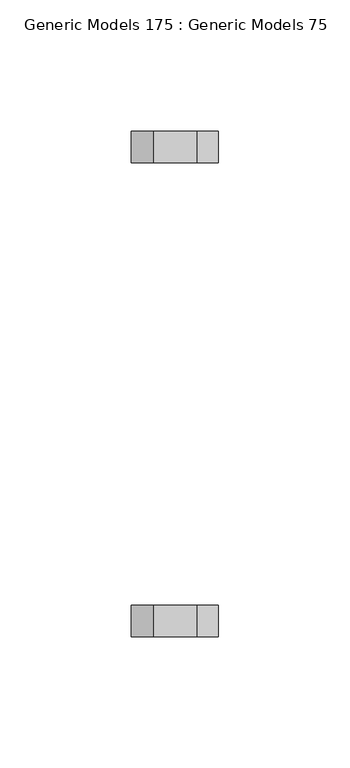
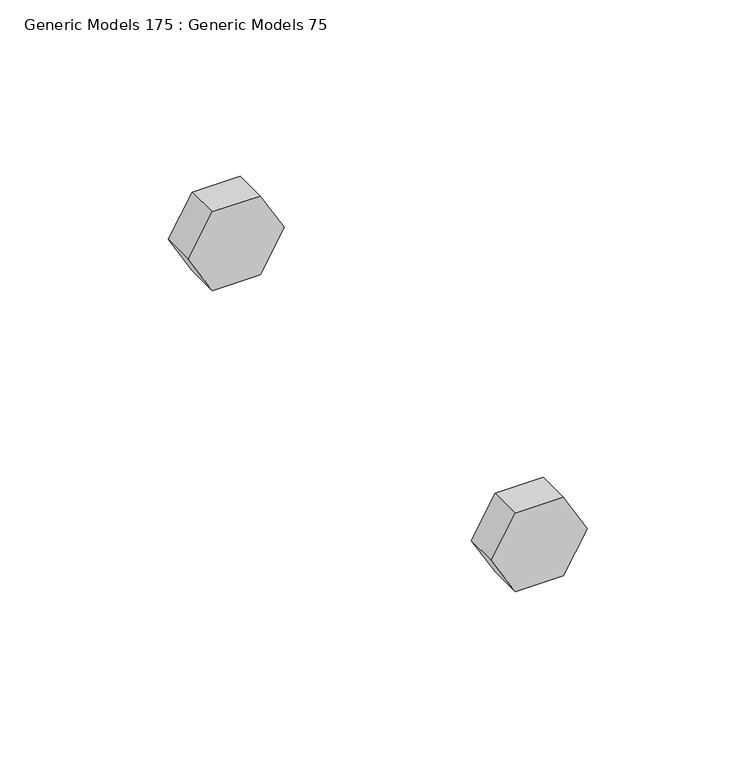
"""IFC4 building model written with IfcOpenShell, lengths in millimetres: proxy geometry, Generic Models 175 : Generic Models 75."""

from ifc_helpers import new_model, si_unit, frame, origin, place, context, project, spatial, polyline, outline, extrude, source, transform, mapped, element, save


def generic_models_175_generic_models_75_4c8c2855(model_context):
    return source(origin(), model_context, "Body", "SweptSolid", [
        extrude(outline(polyline([(271657.7625, 31978.2851858), (271657.7625, 31994.7829698), (271672.05, 32003.0318618), (271686.3375, 31994.7829698), (271686.3375, 31978.2851858), (271672.05, 31970.0362939), (271657.7625, 31978.2851858)])), frame((0.0, 35193.7770442, 0.0), z_axis=(0.0, 1.0, 0.0), x_axis=(0.0, 0.0, 1.0)), (0.0, 0.0, 1.0), 11.90625),
        extrude(outline(polyline([(271657.7625, 31978.2851858), (271657.7625, 31994.7829698), (271672.05, 32003.0318618), (271686.3375, 31994.7829698), (271686.3375, 31978.2851858), (271672.05, 31970.0362939), (271657.7625, 31978.2851858)])), frame((0.0, 35373.9582942, 0.0), z_axis=(0.0, 1.0, 0.0), x_axis=(0.0, 0.0, 1.0)), (0.0, 0.0, 1.0), 11.90625),
    ])


if __name__ == "__main__":
    model = new_model("IFC4")
    model_context = context("Model", 3, world=origin())
    ifc_project = project(units=[si_unit("LENGTHUNIT", "METRE", prefix="MILLI")], contexts=[model_context])
    site = spatial("IfcSite", under=ifc_project)
    building = spatial("IfcBuilding", under=site)
    placement = place(None, origin())
    generic_models_175_generic_models_75_shape = generic_models_175_generic_models_75_4c8c2855(model_context)
    element("IfcBuildingElementProxy", 1, Name="Generic Models 175 : Generic Models 75", ObjectType="Generic Models 175 : Generic Models 75", at=placement, inside=building, context=model_context, shape_type="MappedRepresentation", body=[
        mapped(generic_models_175_generic_models_75_shape, transform((0.0, 0.0, 0.0), x_axis=(1.0, 0.0, 0.0), y_axis=(0.0, 1.0, 0.0), z_axis=(0.0, 0.0, 1.0))),
    ])
    save(model, "model.ifc")

# Revit data of these elements
# Element 1 (IfcBuildingElementProxy, "Generic Models 175 : Generic Models 75")
#   Materials on its faces: "3/4\" GALV. THRU BOLTS"
# Materials
#   "3/4\" GALV. THRU BOLTS": class "Generic", colour RGB 105 69 171, transparency 0, Cost = 0
